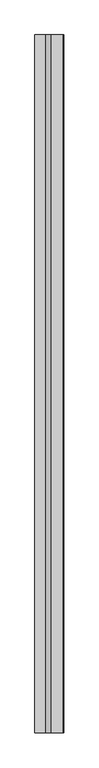
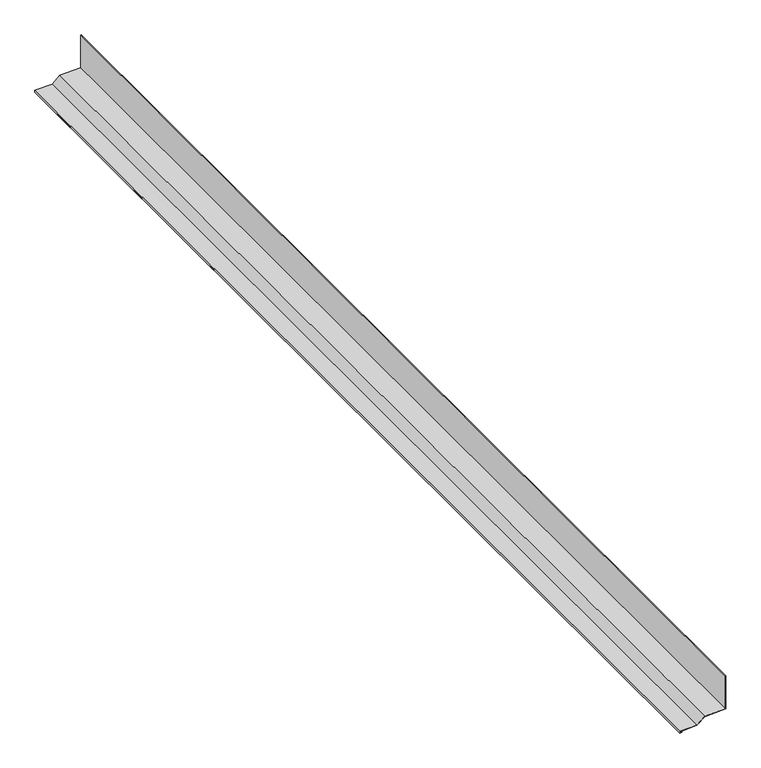
"""IFC4 building model written with IfcOpenShell, lengths in millimetres: proxy geometry, Generic Models 7:Generic Models 1:337419:Generic Models 1:337419 : Generic Models 7:Generic Models 1:337419:28 : Generic Models 7:Generic Models 1:337419:Generic Models 1:337419 : Generic Models 7:Generic Models 1:337419:301336."""

from ifc_helpers import new_model, si_unit, frame, origin, place, context, project, spatial, polyline, outline, extrude, source, transform, mapped, element, save


def generic_models_124643be(model_context):
    return source(origin(), model_context, "Body", "SweptSolid", [
        extrude(outline(polyline([(4847.8534977, 579099.049649), (4844.6812502, 579022.9157088), (4820.1910423, 578993.7294156), (4817.5475027, 578930.2844654), (4811.2030077, 578930.5488194), (4811.5061986, 578937.8254003), (4813.095076, 578937.8254003), (4812.85522, 578932.0688546), (4816.0274675, 578931.9366777), (4818.627426, 578994.3356817), (4843.1176339, 579023.521975), (4846.3307661, 579100.637149), (4974.8534977, 579100.637149), (4974.8534977, 579099.049649), (4847.8534977, 579099.049649)])), frame((0.0, -578778.4413841, 0.0), z_axis=(0.0, 1.0, 0.0), x_axis=(0.0, 0.0, 1.0)), (0.0, 0.0, 1.0), 4126.5124605),
    ])


if __name__ == "__main__":
    model = new_model("IFC4")
    model_context = context("Model", 3, world=origin())
    ifc_project = project(units=[si_unit("LENGTHUNIT", "METRE", prefix="MILLI")], contexts=[model_context])
    site = spatial("IfcSite", under=ifc_project)
    building = spatial("IfcBuilding", under=site)
    placement = place(None, origin())
    generic_models_shape = generic_models_124643be(model_context)
    element("IfcBuildingElementProxy", 1, Name="Generic Models 7:Generic Models 1:337419:Generic Models 1:337419 : Generic Models 7:Generic Models 1:337419:28 : Generic Models 7:Generic Models 1:337419:Generic Models 1:337419 : Generic Models 7:Generic Models 1:337419:301336", ObjectType="Generic Models 7:Generic Models 1:337419:Generic Models 1:337419 : Generic Models 7:Generic Models 1:337419:28 : Generic Models 7:Generic Models 1:337419:Generic Models 1:337419 : Generic Models 7:Generic Models 1:337419:301336", at=placement, inside=building, context=model_context, shape_type="MappedRepresentation", body=[
        mapped(generic_models_shape, transform((0.0, 0.0, 0.0), x_axis=(1.0, 0.0, 0.0), y_axis=(0.0, 1.0, 0.0), z_axis=(0.0, 0.0, 1.0))),
    ])
    save(model, "model.ifc")

# Revit data of these elements
# Type "Generic Models 7:Generic Models 1:337419:Generic Models 1:337419 : Generic Models 7:Generic Models 1:337419:28 : Generic Models 7:Generic Models 1:337419:Generic Models 1:337419 : Generic Models 7:Generic Models 1:337419:301336"
#   NameOverride = "Generic Models 7:Generic Models 1:337419:Generic Models 1:337419 : Generic Models 7:Generic Models 1:337419:301336"
#   ObjectTypeOverride = "Generic Models 1:337419 : Generic Models 7:Generic Models 1:337419"
#   Reference = "Generic Models 1"
#   Tag = "301336"
# Element 1 (IfcBuildingElementProxy, "Generic Models 7:Generic Models 1:337419:Generic Models 1:337419 : Generic Models 7:Generic Models 1:337419:28 : Generic Models 7:Generic Models 1:337419:Generic Models 1:337419 : Generic Models 7:Generic Models 1:337419:301336")
#   Materials on its faces: "BRAKE METAL FLASHING"
# Materials
#   "BRAKE METAL FLASHING": class "Unassigned", colour RGB 210 209 208, transparency 0, Cost = 0
